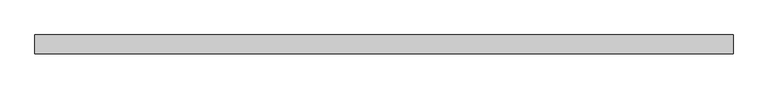
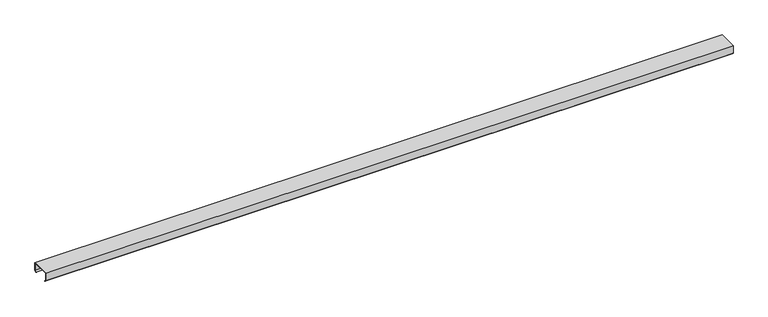
"""IFC4 building model written with IfcOpenShell, lengths in millimetres: proxy geometry, Generic Models 7:Generic Models 1:1:Generic Models 1:1 : Generic Models 7:Generic Models 1:337419:23 : Generic Models 7:Generic Models 1:1:Generic Models 1:1 : Generic Models 7:Generic Models 1:337419:306201."""

from ifc_helpers import new_model, si_unit, frame, origin, place, context, project, spatial, polyline, outline, extrude, source, transform, mapped, element, save


def generic_models_f063353d(model_context):
    return source(origin(), model_context, "Body", "SweptSolid", [
        extrude(outline(polyline([(-578797.4913841, 4985.940625), (-578797.4913841, 4897.040625), (-578812.0845307, 4884.7955211), (-578813.870275, 4886.9236883), (-578800.2695091, 4898.336086), (-578800.2695091, 4983.1625), (-578997.9132591, 4983.1625), (-578997.9132591, 4898.336086), (-578984.3124931, 4886.9236883), (-578986.0982374, 4884.7955211), (-579000.6913841, 4897.040625), (-579000.6913841, 4985.940625), (-578797.4913841, 4985.940625)])), frame((560365.6617239, 0.0, 0.0), z_axis=(1.0, 0.0, 0.0), x_axis=(0.0, 1.0, 0.0)), (0.0, 0.0, 1.0), 7493.0),
    ])


if __name__ == "__main__":
    model = new_model("IFC4")
    model_context = context("Model", 3, world=origin())
    ifc_project = project(units=[si_unit("LENGTHUNIT", "METRE", prefix="MILLI")], contexts=[model_context])
    site = spatial("IfcSite", under=ifc_project)
    building = spatial("IfcBuilding", under=site)
    placement = place(None, origin())
    generic_models_shape = generic_models_f063353d(model_context)
    element("IfcBuildingElementProxy", 1, Name="Generic Models 7:Generic Models 1:1:Generic Models 1:1 : Generic Models 7:Generic Models 1:337419:23 : Generic Models 7:Generic Models 1:1:Generic Models 1:1 : Generic Models 7:Generic Models 1:337419:306201", ObjectType="Generic Models 7:Generic Models 1:1:Generic Models 1:1 : Generic Models 7:Generic Models 1:337419:23 : Generic Models 7:Generic Models 1:1:Generic Models 1:1 : Generic Models 7:Generic Models 1:337419:306201", at=placement, inside=building, context=model_context, shape_type="MappedRepresentation", body=[
        mapped(generic_models_shape, transform((0.0, 0.0, 0.0), x_axis=(1.0, 0.0, 0.0), y_axis=(0.0, 1.0, 0.0), z_axis=(0.0, 0.0, 1.0))),
    ])
    save(model, "model.ifc")

# Revit data of these elements
# Type "Generic Models 7:Generic Models 1:1:Generic Models 1:1 : Generic Models 7:Generic Models 1:337419:23 : Generic Models 7:Generic Models 1:1:Generic Models 1:1 : Generic Models 7:Generic Models 1:337419:306201"
#   NameOverride = "Generic Models 7:Generic Models 1:1:Generic Models 1:1 : Generic Models 7:Generic Models 1:337419:306201"
#   ObjectTypeOverride = "Generic Models 1:1 : Generic Models 7:Generic Models 1:337419"
#   Reference = "Generic Models 1"
#   Tag = "306201"
# Element 1 (IfcBuildingElementProxy, "Generic Models 7:Generic Models 1:1:Generic Models 1:1 : Generic Models 7:Generic Models 1:337419:23 : Generic Models 7:Generic Models 1:1:Generic Models 1:1 : Generic Models 7:Generic Models 1:337419:306201")
#   Materials on its faces: "'ZEE' SECTION (8.0x3.5Z - SEE STRUCT. DWGS)"
# Materials
#   "'ZEE' SECTION (8.0x3.5Z - SEE STRUCT. DWGS)": class "Unassigned", colour RGB 210 209 208, transparency 0, Keynote = "M05121300.02", Cost = 0
